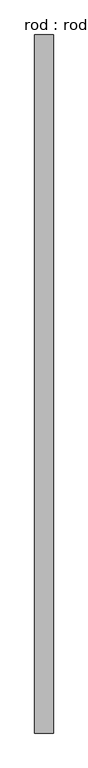
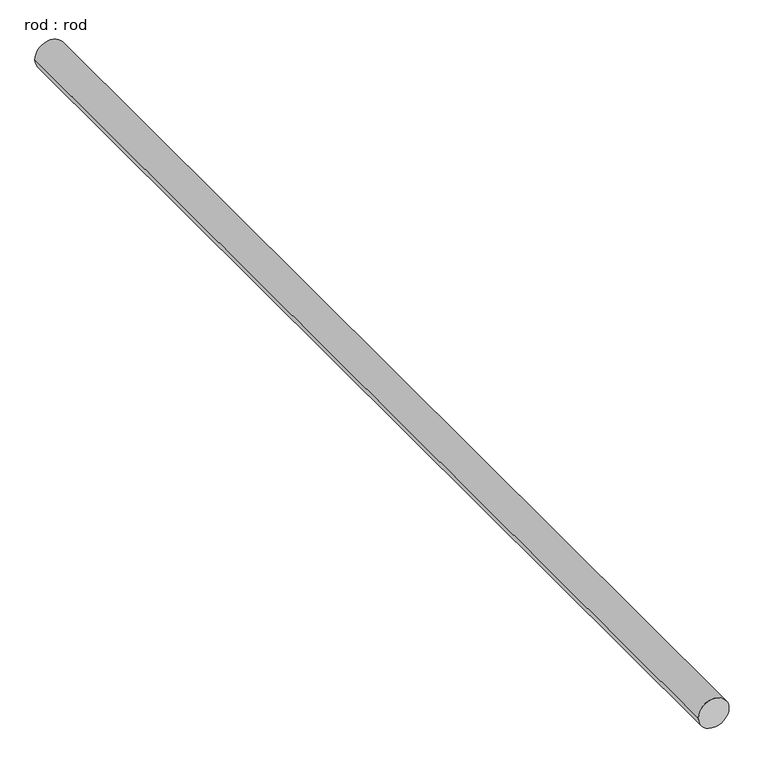
"""IFC4 building model written with IfcOpenShell, lengths in millimetres: proxy geometry, rod : rod."""

from ifc_helpers import new_model, si_unit, point, frame, frame_2d, origin, place, context, project, spatial, circle_curve, trimmed, segment, composite_curve, outline, extrude, source, transform, mapped, element, save


def rod_rod_e87766eb(model_context):
    return source(origin(), model_context, "Body", "SweptSolid", [
        extrude(outline(composite_curve([segment(trimmed(circle_curve(frame_2d((0.0108462, 0.0)), 200.0), [point((0.0108462, 200.0))], [point((0.0108462, -200.0))], False, "CARTESIAN"), True, "CONTINUOUS"), segment(trimmed(circle_curve(frame_2d((0.0108462, 0.0)), 200.0), [point((0.0108462, -200.0))], [point((0.0108462, 200.0))], False, "CARTESIAN"), True, "CONTINUOUS")], self_intersect=False)), frame((0.0, -3396.5453953, 0.0), z_axis=(0.0, 1.0, 0.0), x_axis=(0.0, 0.0, 1.0)), (0.0, 0.0, 1.0), 14978.5480213),
    ])


if __name__ == "__main__":
    model = new_model("IFC4")
    model_context = context("Model", 3, world=origin())
    ifc_project = project(units=[si_unit("LENGTHUNIT", "METRE", prefix="MILLI")], contexts=[model_context])
    site = spatial("IfcSite", under=ifc_project)
    building = spatial("IfcBuilding", under=site)
    placement = place(None, origin())
    rod_rod_shape = rod_rod_e87766eb(model_context)
    element("IfcBuildingElementProxy", 1, Name="rod : rod", ObjectType="rod : rod", at=placement, inside=building, context=model_context, shape_type="MappedRepresentation", body=[
        mapped(rod_rod_shape, transform((0.0, 0.0, 0.0), x_axis=(1.0, 0.0, 0.0), y_axis=(0.0, 1.0, 0.0), z_axis=(0.0, 0.0, 1.0))),
    ])
    save(model, "model.ifc")

# Revit data of these elements
# Type "rod : rod"
#   Default Elevation = 0
